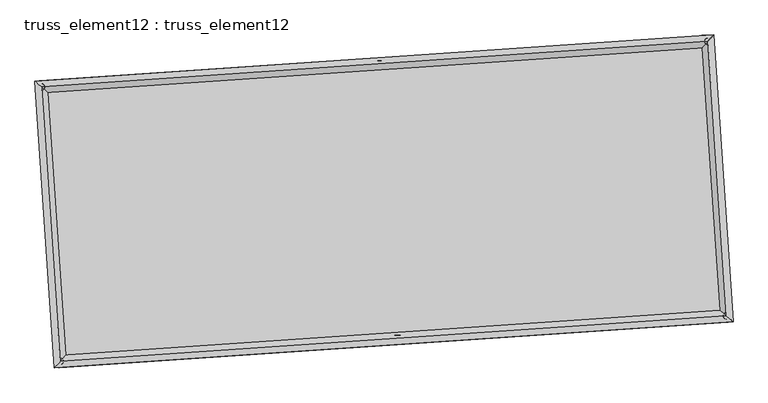
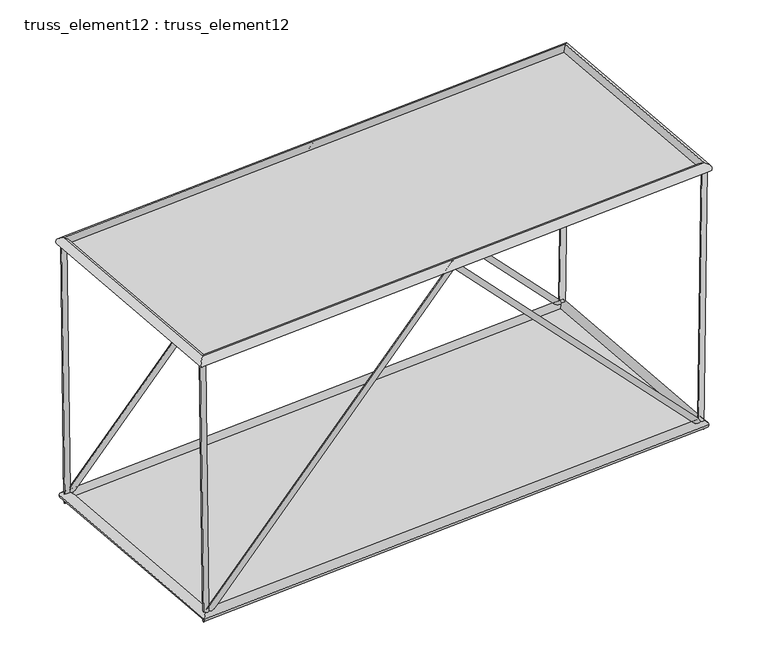
"""IFC4 building model written with IfcOpenShell, lengths in millimetres: plate geometry, truss_element12 : truss_element12."""

import ifcopenshell
import ifcopenshell.guid

model = None  # the IFC model being written
_history = None  # IfcOwnerHistory: only IFC2X3 demands one
_inside = {}  # id of a spatial element -> (the spatial element, [elements in it])
_under = {}  # id of a project, library or spatial element -> (it, [spatial elements below it])
_declared = {}  # id of a project -> (the project, [libraries it declares])
_typed = {}  # id of a type object -> (the type object, [elements of that type])
_made_of = {}  # id of a material, layer set ... -> (it, [elements and type objects made of it])


def new_model(schema):
    """Start an empty IFC model of exactly this schema.

    Asked for "IFC4X3", IfcOpenShell would pick the latest addendum, in which some entities
    have other attributes; the version numbers below select the first issue.
    IFC2X3 requires an IfcOwnerHistory on every rooted entity: one is made here for all.
    """
    global model, _history
    if schema == "IFC4X3":
        model = ifcopenshell.file(schema_version=(4, 3, 0, 0))
    else:
        model = ifcopenshell.file(schema=schema)
    _inside.clear()
    _under.clear()
    _declared.clear()
    _typed.clear()
    _made_of.clear()
    _history = None
    if model.schema == "IFC2X3":
        org = make("IfcOrganization", Name="unknown")
        user = make(
            "IfcPersonAndOrganization",
            ThePerson=make("IfcPerson", FamilyName="unknown"),
            TheOrganization=org,
        )
        app = make(
            "IfcApplication",
            ApplicationDeveloper=org,
            Version="unknown",
            ApplicationFullName="unknown",
            ApplicationIdentifier="unknown",
        )
        _history = make(
            "IfcOwnerHistory",
            OwningUser=user,
            OwningApplication=app,
            ChangeAction="ADDED",
            CreationDate=0,
        )
    return model


def make(cls, **values):
    """One entity of the class cls with the attributes given. An attribute that is None is left unset."""
    return model.create_entity(
        cls, **{name: value for name, value in values.items() if value is not None}
    )


def rooted(cls, **values):
    """An entity with a GlobalId (a new one), such as an element, a storey or a relation."""
    return make(cls, GlobalId=ifcopenshell.guid.new(), OwnerHistory=_history, **values)


def si_unit(unit_type, name, prefix=None):
    """IfcSIUnit, for example si_unit("LENGTHUNIT", "METRE", prefix="MILLI")."""
    return make("IfcSIUnit", UnitType=unit_type, Prefix=prefix, Name=name)


def assignment(units):
    """IfcUnitAssignment: the units of a project."""
    return None if units is None else make("IfcUnitAssignment", Units=units)


def point(xyz):
    """IfcCartesianPoint."""
    return None if xyz is None else make("IfcCartesianPoint", Coordinates=xyz)


def direction(xyz):
    """IfcDirection."""
    return None if xyz is None else make("IfcDirection", DirectionRatios=xyz)


def frame(location, z_axis=None, x_axis=None):
    """IfcAxis2Placement3D, a coordinate frame: its origin and axes. An axis left out is left unset."""
    return make(
        "IfcAxis2Placement3D",
        Location=point(location),
        Axis=direction(z_axis),
        RefDirection=direction(x_axis),
    )


def origin():
    """The frame at (0, 0, 0) with its axes left unset."""
    return frame((0.0, 0.0, 0.0))


def origin_with_axes():
    """The frame at (0, 0, 0) with the z axis (0, 0, 1) and the x axis (1, 0, 0) written out."""
    return frame((0.0, 0.0, 0.0), z_axis=(0.0, 0.0, 1.0), x_axis=(1.0, 0.0, 0.0))


def place(relative_to, where):
    """IfcLocalPlacement: puts the frame where relative to a parent placement (None: the world)."""
    return make(
        "IfcLocalPlacement", PlacementRelTo=relative_to, RelativePlacement=where
    )


def context(
    kind, dimensions, precision=None, world=None, true_north=None, identifier=None
):
    """IfcGeometricRepresentationContext, for example the 3D "Model" context."""
    return make(
        "IfcGeometricRepresentationContext",
        ContextIdentifier=identifier,
        ContextType=kind,
        CoordinateSpaceDimension=dimensions,
        Precision=precision,
        WorldCoordinateSystem=world,
        TrueNorth=true_north,
    )


def project(units=None, contexts=None):
    """IfcProject with its units and contexts."""
    return rooted(
        "IfcProject",
        Name="project",
        RepresentationContexts=contexts,
        UnitsInContext=assignment(units),
    )


def spatial(cls, under=None, at=None, **own):
    """A site, building, storey or space (cls), placed at a placement, below another one or the project."""
    s = rooted(cls, ObjectPlacement=at, **own)
    if under is not None:
        _under.setdefault(under.id(), (under, []))[1].append(s)
    return s


def polyline(points):
    """IfcPolyline through the points."""
    return make("IfcPolyline", Points=[point(p) for p in points])


def circle_curve(where, radius):
    """IfcCircle in the frame where."""
    return make("IfcCircle", Position=where, Radius=radius)


def ellipse_curve(where, semi_axis1, semi_axis2):
    """IfcEllipse in the frame where."""
    return make(
        "IfcEllipse", Position=where, SemiAxis1=semi_axis1, SemiAxis2=semi_axis2
    )


def outline(outer, holes=None, kind="AREA"):
    """IfcArbitraryClosedProfileDef: a profile drawn as a closed curve; with holes, ...WithVoids."""
    if holes is None:
        return make("IfcArbitraryClosedProfileDef", ProfileType=kind, OuterCurve=outer)
    return make(
        "IfcArbitraryProfileDefWithVoids",
        ProfileType=kind,
        OuterCurve=outer,
        InnerCurves=holes,
    )


def extrude(swept, where, along, depth):
    """IfcExtrudedAreaSolid: the profile swept, set in the frame where, extruded along a direction by depth."""
    return make(
        "IfcExtrudedAreaSolid",
        SweptArea=swept,
        Position=where,
        ExtrudedDirection=direction(along),
        Depth=depth,
    )


def shape(context_of_items, identifier, shape_type, items):
    """IfcShapeRepresentation: the items that make up one representation, for example the "Body"."""
    return make(
        "IfcShapeRepresentation",
        ContextOfItems=context_of_items,
        RepresentationIdentifier=identifier,
        RepresentationType=shape_type,
        Items=items,
    )


def source(mapping_origin, context_of_items, identifier, shape_type, items):
    """IfcRepresentationMap: a shape defined once, which mapped items show again and again."""
    return make(
        "IfcRepresentationMap",
        MappingOrigin=mapping_origin,
        MappedRepresentation=shape(context_of_items, identifier, shape_type, items),
    )


def transform(
    local_origin,
    x_axis=None,
    y_axis=None,
    z_axis=None,
    scale=None,
    scale2=None,
    scale3=None,
    uniform=True,
):
    """IfcCartesianTransformationOperator3D, or its non-uniform kind. x_axis, y_axis, z_axis: its Axis1, 2, 3."""
    if uniform:
        return make(
            "IfcCartesianTransformationOperator3D",
            Axis1=direction(x_axis),
            Axis2=direction(y_axis),
            LocalOrigin=point(local_origin),
            Scale=scale,
            Axis3=direction(z_axis),
        )
    return make(
        "IfcCartesianTransformationOperator3DnonUniform",
        Axis1=direction(x_axis),
        Axis2=direction(y_axis),
        LocalOrigin=point(local_origin),
        Scale=scale,
        Axis3=direction(z_axis),
        Scale2=scale2,
        Scale3=scale3,
    )


def mapped(mapping_source, mapping_target):
    """IfcMappedItem: shows the shape of a source again, moved by a transform."""
    return make(
        "IfcMappedItem", MappingSource=mapping_source, MappingTarget=mapping_target
    )


def made_of(thing, what):
    """Note that an element or type object is made of a material, layer set ...; save() writes the relation."""
    if what is not None:
        _made_of.setdefault(what.id(), (what, []))[1].append(thing)
    return thing


def element(
    cls,
    number,
    at=None,
    inside=None,
    cuts=None,
    type_object=None,
    material=None,
    context=None,
    identifier="Body",
    shape_type=None,
    held_by="IfcProductDefinitionShape",
    body=None,
    shapes=None,
    **own,
):
    """One element of the class cls, such as IfcWall. Its Tag is "e" and its number.

    at: its placement. inside: the storey or other place that contains it. cuts: it is an
    opening in that element (IfcRelVoidsElement). A single representation is given by context,
    identifier, shape_type and body (its items); several are given by shapes. held_by: the class
    of the entity that holds the representations. save() writes the other relations.
    """
    e = rooted(cls, Tag="e%d" % number, ObjectPlacement=at, **own)
    if body is not None:
        shapes = [shape(context, identifier, shape_type, body)]
    if shapes is not None:
        e.Representation = make(held_by, Representations=shapes)
    if inside is not None:
        _inside.setdefault(inside.id(), (inside, []))[1].append(e)
    if cuts is not None:
        rooted(
            "IfcRelVoidsElement", RelatingBuildingElement=cuts, RelatedOpeningElement=e
        )
    if type_object is not None:
        _typed.setdefault(type_object.id(), (type_object, []))[1].append(e)
    return made_of(e, material)


def aggregate(whole, parts):
    """IfcRelAggregates: a whole, such as a stair, and the parts it consists of."""
    return rooted("IfcRelAggregates", RelatingObject=whole, RelatedObjects=parts)


def save(model, path):
    """Write the relations noted so far, then the file.

    IfcRelAggregates (storeys below a building ...), IfcRelContainedInSpatialStructure (elements
    in a storey), IfcRelDefinesByType, IfcRelAssociatesMaterial and IfcRelDeclares: one each for
    every whole, place, type object, material and project.
    """
    for whole, parts in _under.values():
        aggregate(whole, parts)
    for where, things in _inside.values():
        rooted(
            "IfcRelContainedInSpatialStructure",
            RelatedElements=things,
            RelatingStructure=where,
        )
    for kind, things in _typed.values():
        rooted("IfcRelDefinesByType", RelatedObjects=things, RelatingType=kind)
    for what, things in _made_of.values():
        rooted("IfcRelAssociatesMaterial", RelatedObjects=things, RelatingMaterial=what)
    for by, libraries in _declared.values():
        rooted("IfcRelDeclares", RelatingContext=by, RelatedDefinitions=libraries)
    model.write(path)


def plane_surface(at):
    """IfcPlane: the flat surface through the origin of the frame at, square to its z axis."""
    return make("IfcPlane", Position=at)


def cylinder_surface(at, radius):
    """IfcCylindricalSurface: all points at the distance radius from the z axis of the frame at."""
    return make("IfcCylindricalSurface", Position=at, Radius=radius)


def advanced_brep(points, edges, surfaces, faces):
    """IfcAdvancedBrep: a solid bounded by faces that lie on surfaces and meet in shared edges.

    An edge is (start, end): straight between two places in points (the first is 0);
    or (start, end, curve); or (start, end, curve, False) where it runs against its curve.
    A face is (place in surfaces, loops), or (place, loops, False) where it looks against
    its surface's normal. A loop lists edges by number (the first is 1), with a minus sign
    where the edge is run from its end to its start. The first loop is the outer one.
    """
    corners = [point(p) for p in points]
    vertices = [make("IfcVertexPoint", VertexGeometry=c) for c in corners]
    made = []
    for start, end, *more in edges:
        made.append(
            make(
                "IfcEdgeCurve",
                EdgeStart=vertices[start],
                EdgeEnd=vertices[end],
                EdgeGeometry=more[0] if more else make("IfcPolyline", Points=[corners[start], corners[end]]),
                SameSense=more[1] if len(more) > 1 else True,
            )
        )
    hull = []
    for where, loops, *sense in faces:
        bounds = []
        for j, loop in enumerate(loops):
            ring = [make("IfcOrientedEdge", EdgeElement=made[abs(k) - 1], Orientation=k > 0) for k in loop]
            bounds.append(
                make(
                    "IfcFaceOuterBound" if j == 0 else "IfcFaceBound",
                    Bound=make("IfcEdgeLoop", EdgeList=ring),
                    Orientation=True,
                )
            )
        hull.append(make("IfcAdvancedFace", Bounds=bounds, FaceSurface=surfaces[where], SameSense=sense[0] if sense else True))
    return make("IfcAdvancedBrep", Outer=make("IfcClosedShell", CfsFaces=hull))


def truss_element12_truss_element12_bcb7a4b1(model_context):
    return source(origin(), model_context, "Body", "SolidModel", [
        advanced_brep(
        [(-3730.6890845, 2271.7408984, 5000.2232822), (-3829.7838055, 2258.3802507, 4998.9082325), (-3666.5483804, 2276.1144092, 122.5077786), (-3762.4385024, 2262.9722709, -122.5077786), (1064.3227767, 2598.6945297, 5071.6784045), (1064.7619686, 2592.1207211, 4927.4371435), (5794.0163085, 2921.1943524, 122.4994051), (5890.7446685, 2921.1861361, -122.4994051), (5859.3257876, 2925.6475575, 5000.2192941), (5959.316593, 2925.861795, 4998.880287)],
        [
            (0, 1, circle_curve(frame((-3780.236445, 2265.0605745, 4999.5657574), z_axis=(-0.013148600710356454, -0.000896553099930443, 0.9999131514746162), x_axis=(-0.13360666404585098, 0.9910340586353044, -0.0008683014310743792)), 50.0)),
            (1, 0, circle_curve(frame((-3780.236445, 2265.0605745, 4999.5657574), z_axis=(-0.013148600710356454, -0.000896553099930443, 0.9999131514746162), x_axis=(-0.13360666404585098, 0.9910340586353044, -0.0008683014310743792)), 50.0)),
            (0, 2),
            (2, 3, ellipse_curve(frame((-3714.4934414, 2269.54334, 0.0), z_axis=(-0.928200365252963, -0.06329045448668467, 0.3666584245795189), x_axis=(0.3658090222339585, 0.024943126655854568, 0.93035563075894)), 131.9651677, 50.0)),
            (3, 1),
            (3, 2, ellipse_curve(frame((-3714.4934414, 2269.54334, 0.0), z_axis=(-0.928200365252963, -0.06329045448668467, 0.3666584245795189), x_axis=(0.3658090222339585, 0.024943126655854568, 0.93035563075894)), 131.9651677, 50.0)),
            (2, 4),
            (4, 5, ellipse_curve(frame((1064.5423727, 2595.4076254, 4999.557774), z_axis=(-0.9976833941197889, -0.06802823809539234, 6.260394869410126e-05), x_axis=(-6.245892014097819e-05, -4.258836334217303e-06, -0.9999999980403728)), 72.2776719, 50.0)),
            (5, 3),
            (5, 4, ellipse_curve(frame((1064.5423727, 2595.4076254, 4999.557774), z_axis=(-0.9976833941197889, -0.06802823809539234, 6.260394869410126e-05), x_axis=(-6.245892014097819e-05, -4.258836334217303e-06, -0.9999999980403728)), 72.2776719, 50.0)),
            (4, 6),
            (6, 7, ellipse_curve(frame((5842.3804885, 2921.1902443, 0.0), z_axis=(-0.9282671693555778, -0.06329500960449407, -0.3664884773846918), x_axis=(-0.36563946873947, -0.02493156544760182, 0.930422589979548)), 131.9466513, 50.0)),
            (7, 5),
            (7, 6, ellipse_curve(frame((5842.3804885, 2921.1902443, 0.0), z_axis=(-0.9282671693555778, -0.06329500960449407, -0.3664884773846918), x_axis=(-0.36563946873947, -0.02493156544760182, 0.930422589979548)), 131.9466513, 50.0)),
            (8, 9, circle_curve(frame((5909.3211903, 2925.7546762, 4999.5497906), z_axis=(0.013388140355829114, 0.0009128863977761105, 0.9999099581143482), x_axis=(-0.002154405773521634, 0.9999972884300797, -0.0008841200433773456)), 50.0)),
            (9, 8, circle_curve(frame((5909.3211903, 2925.7546762, 4999.5497906), z_axis=(0.013388140355829114, 0.0009128863977761105, 0.9999099581143482), x_axis=(-0.002154405773521634, 0.9999972884300797, -0.0008841200433773456)), 50.0)),
            (6, 8),
            (9, 7),
        ],
        [
            plane_surface(frame((-3780.236445, 2315.0605545, 4999.6105889), z_axis=(-0.01314860071035555, -0.000896553099925358, 0.9999131514746165), x_axis=(0.9999135534131738, -1.1789437883713555e-05, 0.01314859542496904))),
            cylinder_surface(frame((-3780.236445, 2265.0605745, 4999.5657574), z_axis=(-0.01314860071035645, -0.0008965530999304427, 0.999913151474616), x_axis=(-0.13360666404585098, 0.9910340586353044, -0.0008683014310743792)), 50.0),
            cylinder_surface(frame((-3714.4934414, 2269.54334, 0.0), z_axis=(-0.6902190995054774, -0.04706341662684533, -0.7220682997426603), x_axis=(-0.02041747777222218, 0.9987519989749245, -0.045580381141596744)), 50.0),
            cylinder_surface(frame((1064.5423727, 2595.4076254, 4999.557774), z_axis=(-0.6901288948828257, -0.04705726591652891, 0.7221549156325607), x_axis=(-0.11534907557209756, 0.9922789741897385, -0.045574424248946074)), 50.0),
            plane_surface(frame((5909.3211903, 2875.7546971, 4999.595439), z_axis=(0.01338814035582826, 0.000912886397775815, 0.9999099581143482), x_axis=(0.9999103748325711, -1.2222946706330628e-05, -0.013388134776246131))),
            cylinder_surface(frame((5842.3804885, 2921.1902443, 0.0), z_axis=(-0.013388140355829114, -0.0009128863977761105, -0.9999099581143482), x_axis=(-0.002154405773521634, 0.9999972884300797, -0.0008841200433773456)), 50.0),
        ],
        [
            (0, [[1, 2]]),
            (1, [[-1, 3, 4, 5]]),
            (1, [[-2, -5, 6, -3]]),
            (2, [[-4, 7, 8, 9]]),
            (2, [[-6, -9, 10, -7]]),
            (3, [[-8, 11, 12, 13]]),
            (3, [[-10, -13, 14, -11]]),
            (4, [[15, 16]]),
            (5, [[-12, 17, -16, 18]]),
            (5, [[-14, -18, -15, -17]]),
        ],
    ),
        advanced_brep(
        [(-3458.5761315, -1718.9926859, 5000.2232822), (-3557.6708526, -1732.3533336, 4998.9082325), (-3394.4354275, -1714.6191751, 122.5077786), (-3490.3255495, -1727.7613134, -122.5077786), (1336.4357296, -1392.0390546, 5071.6784045), (1336.8749216, -1398.6128632, 4927.4371435), (6066.1292614, -1069.5392319, 122.4994051), (6162.8576214, -1069.5474482, -122.4994051), (6131.4387405, -1065.0860268, 5000.2192941), (6231.4295459, -1064.8717893, 4998.880287)],
        [
            (0, 1, circle_curve(frame((-3508.1234921, -1725.6730098, 4999.5657574), z_axis=(-0.013148600710356402, -0.0008965530999304543, 0.9999131514746161), x_axis=(-0.13360666404585028, 0.9910340586353045, -0.0008683014310743518)), 50.0)),
            (1, 0, circle_curve(frame((-3508.1234921, -1725.6730098, 4999.5657574), z_axis=(-0.013148600710356402, -0.0008965530999304543, 0.9999131514746161), x_axis=(-0.13360666404585028, 0.9910340586353045, -0.0008683014310743518)), 50.0)),
            (0, 2),
            (2, 3, ellipse_curve(frame((-3442.3804885, -1721.1902443, 0.0), z_axis=(-0.928200365252963, -0.06329045448668438, 0.36665842457951897), x_axis=(0.36580902223395856, 0.024943126655854433, 0.9303556307589399)), 131.9651677, 50.0)),
            (3, 1),
            (3, 2, ellipse_curve(frame((-3442.3804885, -1721.1902443, 0.0), z_axis=(-0.928200365252963, -0.06329045448668438, 0.36665842457951897), x_axis=(0.36580902223395856, 0.024943126655854433, 0.9303556307589399)), 131.9651677, 50.0)),
            (2, 4),
            (4, 5, ellipse_curve(frame((1336.6553256, -1395.3259589, 4999.557774), z_axis=(-0.997683394119789, -0.06802823809539227, 6.260394869466301e-05), x_axis=(-6.245892014143939e-05, -4.258836333986682e-06, -0.9999999980403728)), 72.2776719, 50.0)),
            (5, 3),
            (5, 4, ellipse_curve(frame((1336.6553256, -1395.3259589, 4999.557774), z_axis=(-0.997683394119789, -0.06802823809539227, 6.260394869466301e-05), x_axis=(-6.245892014143939e-05, -4.258836333986682e-06, -0.9999999980403728)), 72.2776719, 50.0)),
            (4, 6),
            (6, 7, ellipse_curve(frame((6114.4934414, -1069.54334, 0.0), z_axis=(-0.9282671693555782, -0.06329500960449432, -0.36648847738469165), x_axis=(-0.3656394687394694, -0.02493156544760184, 0.9304225899795483)), 131.9466513, 50.0)),
            (7, 5),
            (7, 6, ellipse_curve(frame((6114.4934414, -1069.54334, 0.0), z_axis=(-0.9282671693555782, -0.06329500960449432, -0.36648847738469165), x_axis=(-0.3656394687394694, -0.02493156544760184, 0.9304225899795483)), 131.9466513, 50.0)),
            (8, 9, circle_curve(frame((6181.4341432, -1064.9789081, 4999.5497906), z_axis=(0.013388140355828559, 0.0009128863977761051, 0.9999099581143482), x_axis=(-0.0021544057735223424, 0.9999972884300797, -0.0008841200433773321)), 50.0)),
            (9, 8, circle_curve(frame((6181.4341432, -1064.9789081, 4999.5497906), z_axis=(0.013388140355828559, 0.0009128863977761051, 0.9999099581143482), x_axis=(-0.0021544057735223424, 0.9999972884300797, -0.0008841200433773321)), 50.0)),
            (6, 8),
            (9, 7),
        ],
        [
            plane_surface(frame((-3508.1234921, -1675.6730298, 4999.6105889), z_axis=(-0.01314860071035555, -0.0008965530999253677, 0.9999131514746165), x_axis=(0.9999135534131738, -1.1789437883713555e-05, 0.01314859542496904))),
            cylinder_surface(frame((-3508.1234921, -1725.6730098, 4999.5657574), z_axis=(-0.013148600710356402, -0.0008965530999304543, 0.9999131514746161), x_axis=(-0.13360666404585028, 0.9910340586353045, -0.0008683014310743518)), 50.0),
            cylinder_surface(frame((-3442.3804885, -1721.1902443, 0.0), z_axis=(-0.6902190995054773, -0.04706341662684507, -0.7220682997426601), x_axis=(-0.020417477772222078, 0.9987519989749246, -0.0455803811415965)), 50.0),
            cylinder_surface(frame((1336.6553256, -1395.3259589, 4999.557774), z_axis=(-0.6901288948828249, -0.04705726591652899, 0.7221549156325613), x_axis=(-0.11534907557209753, 0.9922789741897384, -0.045574424248945776)), 50.0),
            plane_surface(frame((6181.4341432, -1114.9788872, 4999.595439), z_axis=(0.013388140355828259, 0.0009128863977758237, 0.9999099581143482), x_axis=(0.9999103748325711, -1.2222946705886538e-05, -0.013388134776246131))),
            cylinder_surface(frame((6114.4934414, -1069.54334, 0.0), z_axis=(-0.013388140355828559, -0.0009128863977761051, -0.9999099581143482), x_axis=(-0.0021544057735223424, 0.9999972884300797, -0.0008841200433773321)), 50.0),
        ],
        [
            (0, [[1, 2]]),
            (1, [[-1, 3, 4, 5]]),
            (1, [[-2, -5, 6, -3]]),
            (2, [[-4, 7, 8, 9]]),
            (2, [[-6, -9, 10, -7]]),
            (3, [[-8, 11, 12, 13]]),
            (3, [[-10, -13, 14, -11]]),
            (4, [[15, 16]]),
            (5, [[-12, 17, -16, 18]]),
            (5, [[-14, -18, -15, -17]]),
        ],
    ),
        advanced_brep(
        [(-3508.127679, -1725.6776503, 4909.5657575), (-3508.1193051, -1725.6683692, 5089.5657573), (-3780.2316669, 2265.0565453, 5089.5657573), (-3780.2412231, 2265.0646038, 4909.5657575), (5909.3172986, 2925.7500558, 5089.5497905), (5909.325082, 2925.7592967, 4909.5497907), (6181.4296603, -1064.9748587, 5089.5497905), (6181.4386261, -1064.9829574, 4909.5497907)],
        [
            (0, 1, ellipse_curve(frame((-3508.1234921, -1725.6730098, 4999.5657574), z_axis=(-0.7535719234045049, 0.6573654662781456, 1.1624966694194113e-06), x_axis=(-0.6573654662771273, -0.753571923405393, 1.1624966755451343e-06)), 127.2792206, 90.0)),
            (1, 2),
            (2, 3, ellipse_curve(frame((-3780.236445, 2265.0605745, 4999.5657574), z_axis=(-0.6573654662771272, -0.753571923405393, 1.1624966742049372e-06), x_axis=(0.7535719234045045, -0.6573654662781458, -1.162496668079214e-06)), 127.2792206, 90.0)),
            (3, 0),
            (1, 0, ellipse_curve(frame((-3508.1234921, -1725.6730098, 4999.5657574), z_axis=(-0.7535719234045049, 0.6573654662781456, 1.1624966694194113e-06), x_axis=(-0.6573654662771273, -0.753571923405393, 1.1624966755451343e-06)), 127.2792206, 90.0)),
            (3, 2, ellipse_curve(frame((-3780.236445, 2265.0605745, 4999.5657574), z_axis=(-0.6573654662771272, -0.753571923405393, 1.1624966742049372e-06), x_axis=(0.7535719234045045, -0.6573654662781458, -1.162496668079214e-06)), 127.2792206, 90.0)),
            (2, 4),
            (4, 5, ellipse_curve(frame((5909.3211903, 2925.7546762, 4999.5497906), z_axis=(-0.7535719234045039, 0.6573654662781465, 1.1624966713335448e-06), x_axis=(-0.6573654662771284, -0.7535719234053921, 1.1624966709506072e-06)), 127.2792206, 90.0)),
            (5, 3),
            (5, 4, ellipse_curve(frame((5909.3211903, 2925.7546762, 4999.5497906), z_axis=(-0.7535719234045039, 0.6573654662781465, 1.1624966713335448e-06), x_axis=(-0.6573654662771284, -0.7535719234053921, 1.1624966709506072e-06)), 127.2792206, 90.0)),
            (4, 6),
            (6, 7, ellipse_curve(frame((6181.4341432, -1064.9789081, 4999.5497906), z_axis=(0.6573654662771281, 0.7535719234053923, -1.1624966722908037e-06), x_axis=(-0.7535719234045039, 0.6573654662781466, 1.1624966726737413e-06)), 127.2792206, 90.0)),
            (7, 5),
            (7, 6, ellipse_curve(frame((6181.4341432, -1064.9789081, 4999.5497906), z_axis=(0.6573654662771281, 0.7535719234053923, -1.1624966722908037e-06), x_axis=(-0.7535719234045039, 0.6573654662781466, 1.1624966726737413e-06)), 127.2792206, 90.0)),
            (6, 1),
            (0, 7),
        ],
        [
            cylinder_surface(frame((-3508.1234921, -1725.6730098, 4999.5657574), z_axis=(0.06802823822870312, -0.9976833960748764, 0.0), x_axis=(-0.9976833948316876, -0.0680282381439348, 4.9921449588598364e-05)), 90.0),
            cylinder_surface(frame((-3780.236445, 2265.0605745, 4999.5657574), z_axis=(-0.9976833960735286, -0.06802823822860814, 1.6440185585427e-06), x_axis=(-0.06802823807023788, 0.9976833949176206, 4.8277431027640126e-05)), 90.0),
            cylinder_surface(frame((5909.3211903, 2925.7546762, 4999.5497906), z_axis=(-0.0680282382287005, 0.9976833960748769, 0.0), x_axis=(0.9976833949900581, 0.06802823815473083, 4.663341247074265e-05)), 90.0),
            cylinder_surface(frame((6181.4341432, -1064.9789081, 4999.5497906), z_axis=(0.9976833960735284, 0.06802823822860798, -1.6440185604380239e-06), x_axis=(0.06802823822860797, -0.9976833949068218, 4.8277431028994146e-05)), 90.0),
        ],
        [
            (0, [[1, 2, 3, 4]]),
            (0, [[5, -4, 6, -2]]),
            (1, [[-3, 7, 8, 9]]),
            (1, [[-6, -9, 10, -7]]),
            (2, [[-8, 11, 12, 13]]),
            (2, [[-10, -13, 14, -11]]),
            (3, [[-12, 15, -1, 16]]),
            (3, [[-14, -16, -5, -15]]),
        ],
    ),
        advanced_brep(
        [(-3358.7115243, -1625.2761972, 0.0), (-3526.0494527, -1817.1042913, 0.0), (-3810.4074885, 2353.2123043, 0.0), (-3618.5793943, 2185.8743758, 0.0), (5926.0494527, 3017.1042913, 0.0), (5758.7115243, 2825.2761972, 0.0), (6210.4074885, -1153.2123043, 0.0), (6018.5793943, -985.8743758, 0.0)],
        [
            (0, 1, ellipse_curve(frame((-3442.3804885, -1721.1902443, 0.0), z_axis=(-0.7535719234054598, 0.6573654662780787, 0.0), x_axis=(-0.6573654662780786, -0.7535719234054599, 0.0)), 127.2792206, 90.0)),
            (1, 2),
            (2, 3, ellipse_curve(frame((-3714.4934414, 2269.54334, 0.0), z_axis=(-0.6573654662780787, -0.7535719234054596, 0.0), x_axis=(0.7535719234054594, -0.657365466278079, 0.0)), 127.2792206, 90.0)),
            (3, 0),
            (1, 0, ellipse_curve(frame((-3442.3804885, -1721.1902443, 0.0), z_axis=(-0.7535719234054598, 0.6573654662780787, 0.0), x_axis=(-0.6573654662780786, -0.7535719234054599, 0.0)), 127.2792206, 90.0)),
            (3, 2, ellipse_curve(frame((-3714.4934414, 2269.54334, 0.0), z_axis=(-0.6573654662780787, -0.7535719234054596, 0.0), x_axis=(0.7535719234054594, -0.657365466278079, 0.0)), 127.2792206, 90.0)),
            (2, 4),
            (4, 5, ellipse_curve(frame((5842.3804885, 2921.1902443, 0.0), z_axis=(-0.7535719234054591, 0.6573654662780796, 0.0), x_axis=(-0.6573654662780795, -0.753571923405459, 0.0)), 127.2792206, 90.0)),
            (5, 3),
            (5, 4, ellipse_curve(frame((5842.3804885, 2921.1902443, 0.0), z_axis=(-0.7535719234054591, 0.6573654662780796, 0.0), x_axis=(-0.6573654662780795, -0.753571923405459, 0.0)), 127.2792206, 90.0)),
            (4, 6),
            (6, 7, ellipse_curve(frame((6114.4934414, -1069.54334, 0.0), z_axis=(0.6573654662780797, 0.7535719234054589, 0.0), x_axis=(-0.7535719234054589, 0.6573654662780799, 0.0)), 127.2792206, 90.0)),
            (7, 5),
            (7, 6, ellipse_curve(frame((6114.4934414, -1069.54334, 0.0), z_axis=(0.6573654662780797, 0.7535719234054589, 0.0), x_axis=(-0.7535719234054589, 0.6573654662780799, 0.0)), 127.2792206, 90.0)),
            (6, 1),
            (0, 7),
        ],
        [
            cylinder_surface(frame((-3442.3804885, -1721.1902443, 0.0), z_axis=(0.06802823822870559, -0.9976833960748764, 0.0), x_axis=(-0.9976833960748764, -0.06802823822870559, 0.0)), 90.0),
            cylinder_surface(frame((-3714.4934414, 2269.54334, 0.0), z_axis=(-0.9976833960748767, -0.06802823822870269, 0.0), x_axis=(-0.06802823822870269, 0.9976833960748767, 0.0)), 90.0),
            cylinder_surface(frame((5842.3804885, 2921.1902443, 0.0), z_axis=(-0.068028238228703, 0.9976833960748764, 0.0), x_axis=(0.9976833960748764, 0.068028238228703, 0.0)), 90.0),
            cylinder_surface(frame((6114.4934414, -1069.54334, 0.0), z_axis=(0.9976833960748765, 0.06802823822870231, 0.0), x_axis=(0.06802823822870231, -0.9976833960748765, 0.0)), 90.0),
        ],
        [
            (0, [[1, 2, 3, 4]]),
            (0, [[5, -4, 6, -2]]),
            (1, [[-3, 7, 8, 9]]),
            (1, [[-6, -9, 10, -7]]),
            (2, [[-8, 11, 12, 13]]),
            (2, [[-10, -13, 14, -11]]),
            (3, [[-12, 15, -1, 16]]),
            (3, [[-14, -16, -5, -15]]),
        ],
    ),
        extrude(outline(polyline([(-3442.3804885, -1721.1902443), (-3714.4934414, 2269.54334), (5842.3804885, 2921.1902443), (6114.4934414, -1069.54334), (-3442.3804885, -1721.1902443)])), origin_with_axes(), (0.0, 0.0, 1.0), 20.0),
        extrude(outline(polyline([(-2000.0, 4856.0283119), (2000.0, 4856.0283119), (2000.0, -4856.0283119), (-2000.0, -4856.0283119), (-2000.0, 4856.0283119)])), frame((1200.5988491, 600.0408332, 4999.557774), z_axis=(1.6402100184022758e-06, 1.1183969047438534e-07, 0.9999999999986487), x_axis=(-0.06802823822870536, 0.9976833960748763, 0.0)), (0.0, 0.0, 1.0), 20.0),
    ])


if __name__ == "__main__":
    model = new_model("IFC4")
    model_context = context("Model", 3, world=origin())
    ifc_project = project(units=[si_unit("LENGTHUNIT", "METRE", prefix="MILLI")], contexts=[model_context])
    site = spatial("IfcSite", under=ifc_project)
    building = spatial("IfcBuilding", under=site)
    placement = place(None, origin())
    truss_element12_truss_element12_shape = truss_element12_truss_element12_bcb7a4b1(model_context)
    element("IfcPlate", 1, ObjectType="truss_element12 : truss_element12", at=placement, inside=building, context=model_context, shape_type="MappedRepresentation", body=[
        mapped(truss_element12_truss_element12_shape, transform((0.0, 0.0, 0.0), x_axis=(1.0, 0.0, 0.0), y_axis=(0.0, 1.0, 0.0), z_axis=(0.0, 0.0, 1.0))),
    ])
    save(model, "model.ifc")

# Revit data of these elements
# Type "truss_element12 : truss_element12"
#   steellbar1 = 90 mm
#   steelbar2 = 50 mm
#   offset1 = 5000 mm
#   M = Default Roof
# Element 1 (IfcPlate, "truss_element12 : truss_element12")
#   Materials on its faces: "Default Roof"
# Materials
#   "Default Roof": class "Miscellaneous", colour RGB 0 127 0, transparency 0, Comments = "Rendering appearance not upgraded Rendering appearance not upgraded ", Cost = 0
